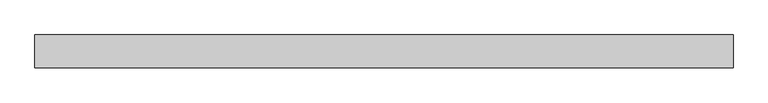
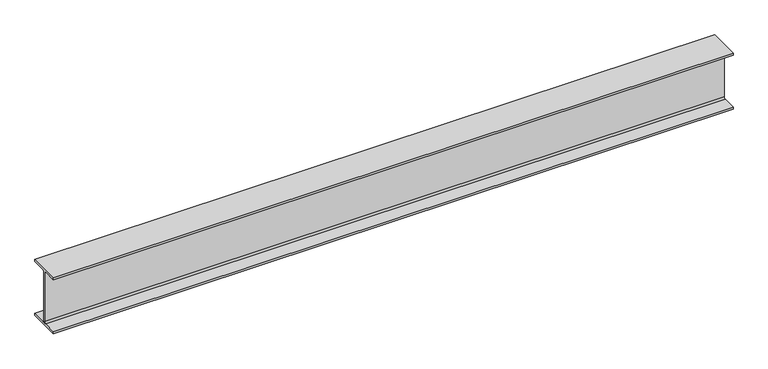
"""IFC4 building model written with IfcOpenShell, lengths in millimetres: beam geometry, Old_Steel Beam_H-KSD3502 : H_SB_ASB_H-200×200x8x12."""

from ifc_helpers import new_model, si_unit, point, frame, frame_2d, origin, place, context, project, spatial, polyline, circle_curve, trimmed, segment, composite_curve, outline, extrude, source, transform, mapped, element, save


def beam_15c682c9(model_context):
    return source(origin(), model_context, "Body", "SweptSolid", [
        extrude(outline(composite_curve([segment(polyline([(82.5, -141.5), (82.5, -151.7), (-82.5, -151.7), (-82.5, -141.5), (-11.9, -141.5)]), True, "CONTINUOUS"), segment(trimmed(circle_curve(frame_2d((-11.9, -132.6)), 8.9), [point((-11.9, -141.5))], [point((-3.0, -132.6))], True, "CARTESIAN"), True, "CONTINUOUS"), segment(polyline([(-3.0, -132.6), (-3.0, 132.6)]), True, "CONTINUOUS"), segment(trimmed(circle_curve(frame_2d((-11.9, 132.6)), 8.9), [point((-3.0, 132.6))], [point((-11.9, 141.5))], True, "CARTESIAN"), True, "CONTINUOUS"), segment(polyline([(-11.9, 141.5), (-82.5, 141.5), (-82.5, 151.7), (82.5, 151.7), (82.5, 141.5), (11.9, 141.5)]), True, "CONTINUOUS"), segment(trimmed(circle_curve(frame_2d((11.9, 132.6)), 8.9), [point((11.9, 141.5))], [point((3.0, 132.6))], True, "CARTESIAN"), True, "CONTINUOUS"), segment(polyline([(3.0, 132.6), (3.0, -132.6)]), True, "CONTINUOUS"), segment(trimmed(circle_curve(frame_2d((11.9, -132.6)), 8.9), [point((3.0, -132.6))], [point((11.9, -141.5))], True, "CARTESIAN"), True, "CONTINUOUS"), segment(polyline([(11.9, -141.5), (82.5, -141.5)]), True, "CONTINUOUS")], self_intersect=False)), frame((-1797.1435209, 0.0, 0.0), z_axis=(1.0, 0.0, 0.0), x_axis=(0.0, 1.0, 0.0)), (0.0, 0.0, 1.0), 3494.7665712),
    ])


if __name__ == "__main__":
    model = new_model("IFC4")
    model_context = context("Model", 3, world=origin())
    ifc_project = project(units=[si_unit("LENGTHUNIT", "METRE", prefix="MILLI")], contexts=[model_context])
    site = spatial("IfcSite", under=ifc_project)
    building = spatial("IfcBuilding", under=site)
    placement = place(None, origin())
    beam_shape = beam_15c682c9(model_context)
    element("IfcBeam", 1, ObjectType="Old_Steel Beam_H-KSD3502 : H_SB_ASB_H-200×200x8x12", at=placement, inside=building, context=model_context, shape_type="MappedRepresentation", body=[
        mapped(beam_shape, transform((0.0, 0.0, 0.0), x_axis=(1.0, 0.0, 0.0), y_axis=(0.0, 1.0, 0.0), z_axis=(0.0, 0.0, 1.0))),
    ])
    save(model, "model.ifc")

# Revit data of these elements
# Type "Old_Steel Beam_H-KSD3502 : H_SB_ASB_H-200×200x8x12"
#   Width = 20.0 cm
#   Web Thickness = 0.8 cm
#   Web Fillet = 1.3 cm
#   Warping Constant = 141376.0 cm⁶
#   Torsional Moment of Inertia = 26.2485 cm⁴
#   Torsional Modulus = 1.0 cm³
#   Section Area = 63.53 cm²
#   Plastic Modulus weak axis = 244.0 cm³
#   Plastic Modulus strong axis = 525.0 cm³
#   Perimeter = 1.16 m²/m
#   Nominal Weight = 49.90 kgf/m
#   Moment of Inertia weak axis = 1600.00 cm⁴
#   Moment of Inertia strong axis = 4720.00 cm⁴
#   Height = 20.0 cm
#   Flange Thickness = 1.2 cm
#   Elastic Modulus weak axis = 160.0 cm³
#   Elastic Modulus strong axis = 472.0 cm³
#   Centroid Vertical = 10.0 cm
#   Centroid Horizontal = 10.0 cm
#   Length [instance default] = 1.5240 m
#   Structural Material [instance default] = Steel, 45-345
#   Assembly Code = ""
# Element 1 (IfcBeam, "Old_Steel Beam_H-KSD3502 : H_SB_ASB_H-200×200x8x12")
#   Structural Material = none
# Materials
#   "Steel, 45-345": class "Metal", colour RGB 189 187 185, transparency 0, Description = "Steel 345 MPa", Cost = 0
